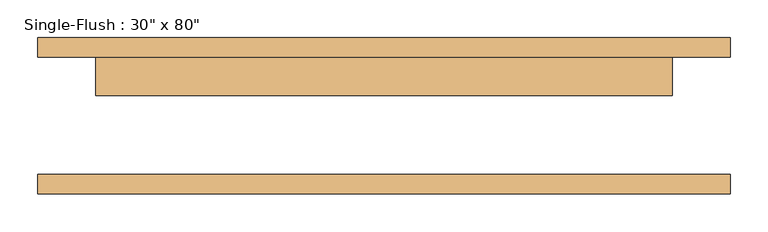
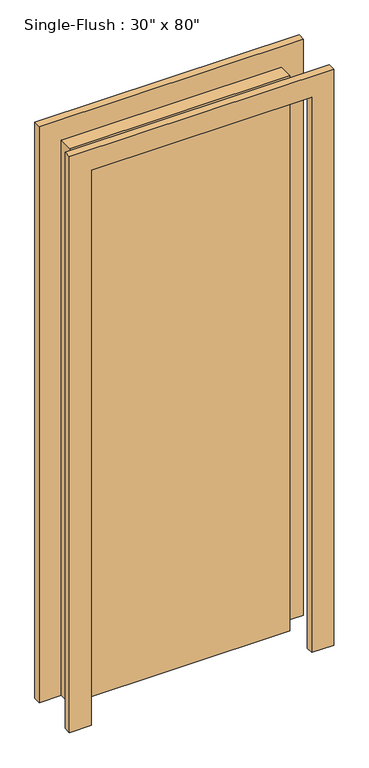
"""IFC4 building model written with IfcOpenShell, lengths in millimetres: door geometry."""

from ifc_helpers import new_model, si_unit, frame, origin, origin_with_axes, place, context, project, spatial, polyline, outline, extrude, source, transform, mapped, element, save


def door_a57ad9fa(model_context):
    return source(origin(), model_context, "Body", "SweptSolid", [
        extrude(outline(polyline([(2108.2, -457.2), (0.0, -457.2), (0.0, -381.0), (2032.0, -381.0), (2032.0, 381.0), (0.0, 381.0), (0.0, 457.2), (2108.2, 457.2), (2108.2, -457.2)])), frame((0.0, 77.7875, 0.0), z_axis=(0.0, 1.0, 0.0), x_axis=(0.0, 0.0, 1.0)), (0.0, 0.0, 1.0), 25.4),
        extrude(outline(polyline([(2108.2, 457.2), (2108.2, -457.2), (0.0, -457.2), (0.0, -381.0), (2032.0, -381.0), (2032.0, 381.0), (0.0, 381.0), (0.0, 457.2), (2108.2, 457.2)])), frame((0.0, -103.1875, 0.0), z_axis=(0.0, 1.0, 0.0), x_axis=(0.0, 0.0, 1.0)), (0.0, 0.0, 1.0), 25.4),
        extrude(outline(polyline([(381.0, 26.9875), (-381.0, 26.9875), (-381.0, 77.7875), (381.0, 77.7875), (381.0, 26.9875)])), origin_with_axes(), (0.0, 0.0, 1.0), 2032.0),
    ])


if __name__ == "__main__":
    model = new_model("IFC4")
    model_context = context("Model", 3, world=origin())
    ifc_project = project(units=[si_unit("LENGTHUNIT", "METRE", prefix="MILLI")], contexts=[model_context])
    site = spatial("IfcSite", under=ifc_project)
    building = spatial("IfcBuilding", under=site)
    placement = place(None, origin())
    door_shape = door_a57ad9fa(model_context)
    element("IfcDoor", 1, ObjectType="Single-Flush : 30\" x 80\"", at=placement, inside=building, context=model_context, shape_type="MappedRepresentation", body=[
        mapped(door_shape, transform((0.0, 0.0, 0.0), x_axis=(1.0, 0.0, 0.0), y_axis=(0.0, 1.0, 0.0), z_axis=(0.0, 0.0, 1.0))),
    ])
    save(model, "model.ifc")

# Revit data of these elements
# Type "Single-Flush : 30\" x 80\""
#   Type Mark = "5"
#   Construction Type Id = "MDOOR"
#   Assembly Code = "C1020"
#   Analytic Construction = "Metal"
#   Thickness = 0' - 2"
#   Heat Transfer Coefficient (U) = 3.7021 W/(m²·K)
#   Height = 6' - 8"
#   Trim Projection Ext = 0' - 1"
#   Trim Projection Int = 0' - 1"
#   Trim Width = 0' - 3"
#   Width = 2' - 6"
#   Door Material = Door - Panel
#   Frame Material = Door - Frame
#   Visual Light Transmittance = 0
#   Solar Heat Gain Coefficient = 0
#   Function = (empty or 0)
#   Wall Closure = (empty or 0)
# Element 1 (IfcDoor, "Single-Flush : 30\" x 80\"")
#   Materials on its faces: "Door - Frame", "Door - Panel"
# Materials
#   "Door - Panel": class "Wood", colour RGB 210 159 95, transparency 0, Cost = 0
#   "Door - Frame": class "Miscellaneous", colour RGB 118 70 51, transparency 0, Cost = 0
